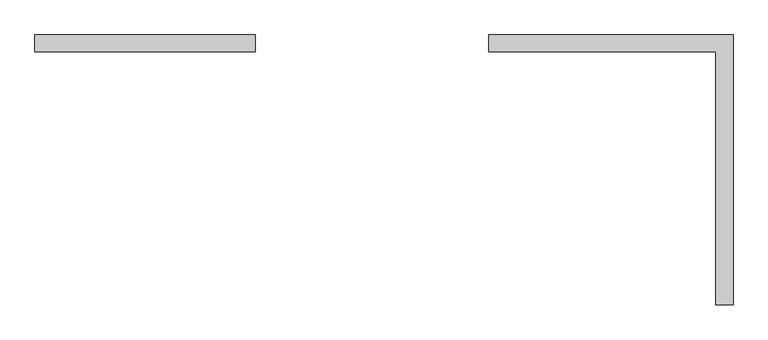
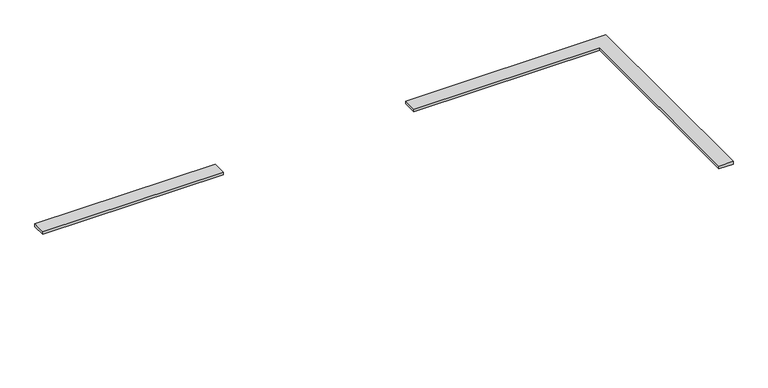
"""IFC4 building model written with IfcOpenShell, lengths in millimetres: furniture geometry, Bridge - Left Uper : Bridge - Left Uper."""

from ifc_helpers import new_model, si_unit, frame, origin, place, context, project, spatial, polyline, outline, extrude, source, transform, mapped, element, save


def furniture_50efe6d3(model_context):
    return source(origin(), model_context, "Body", "SweptSolid", [
        extrude(outline(polyline([(3702.05, 11963.4), (3702.05, 9931.4), (3571.1056594, 9931.4), (3571.1056594, 11836.4), (1860.55, 11836.4), (1860.55, 11963.4), (3702.05, 11963.4)])), frame((0.0, 0.0, 3041.65), z_axis=(0.0, 0.0, 1.0), x_axis=(1.0, 0.0, 0.0)), (0.0, 0.0, 1.0), 25.4),
        extrude(outline(polyline([(-1557.667512, 11963.4), (103.1875, 11963.4), (103.1875, 11836.4), (-1557.667512, 11836.4), (-1557.667512, 11963.4)])), frame((0.0, 0.0, 3041.65), z_axis=(0.0, 0.0, 1.0), x_axis=(1.0, 0.0, 0.0)), (0.0, 0.0, 1.0), 25.4),
    ])


if __name__ == "__main__":
    model = new_model("IFC4")
    model_context = context("Model", 3, world=origin())
    ifc_project = project(units=[si_unit("LENGTHUNIT", "METRE", prefix="MILLI")], contexts=[model_context])
    site = spatial("IfcSite", under=ifc_project)
    building = spatial("IfcBuilding", under=site)
    placement = place(None, origin())
    furniture_shape = furniture_50efe6d3(model_context)
    element("IfcFurniture", 1, ObjectType="Bridge - Left Uper : Bridge - Left Uper", at=placement, inside=building, context=model_context, shape_type="MappedRepresentation", body=[
        mapped(furniture_shape, transform((0.0, 0.0, 0.0), x_axis=(1.0, 0.0, 0.0), y_axis=(0.0, 1.0, 0.0), z_axis=(0.0, 0.0, 1.0))),
    ])
    save(model, "model.ifc")

# Revit data of these elements
# Type "Bridge - Left Uper : Bridge - Left Uper"
#   COBie.Type = no
# Element 1 (IfcFurniture, "Bridge - Left Uper : Bridge - Left Uper")
#   Materials on its faces: "Trim - White"
# Materials
#   "Trim - White": class "Wood", colour RGB 255 255 255, transparency 0, Cost = 0
